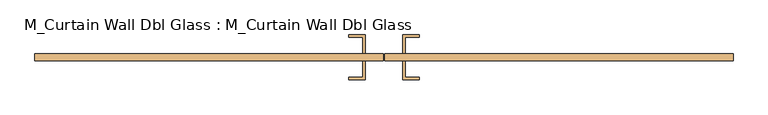
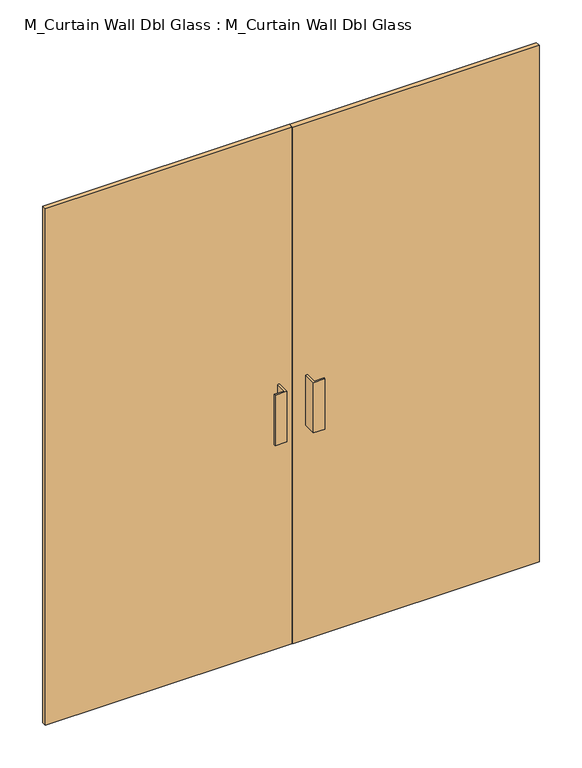
"""IFC4 building model written with IfcOpenShell, lengths in millimetres: door geometry, M_Curtain Wall Dbl Glass : M_Curtain Wall Dbl Glass."""

import ifcopenshell
import ifcopenshell.guid

model = None  # the IFC model being written
_history = None  # IfcOwnerHistory: only IFC2X3 demands one
_inside = {}  # id of a spatial element -> (the spatial element, [elements in it])
_under = {}  # id of a project, library or spatial element -> (it, [spatial elements below it])
_declared = {}  # id of a project -> (the project, [libraries it declares])
_typed = {}  # id of a type object -> (the type object, [elements of that type])
_made_of = {}  # id of a material, layer set ... -> (it, [elements and type objects made of it])


def new_model(schema):
    """Start an empty IFC model of exactly this schema.

    Asked for "IFC4X3", IfcOpenShell would pick the latest addendum, in which some entities
    have other attributes; the version numbers below select the first issue.
    IFC2X3 requires an IfcOwnerHistory on every rooted entity: one is made here for all.
    """
    global model, _history
    if schema == "IFC4X3":
        model = ifcopenshell.file(schema_version=(4, 3, 0, 0))
    else:
        model = ifcopenshell.file(schema=schema)
    _inside.clear()
    _under.clear()
    _declared.clear()
    _typed.clear()
    _made_of.clear()
    _history = None
    if model.schema == "IFC2X3":
        org = make("IfcOrganization", Name="unknown")
        user = make(
            "IfcPersonAndOrganization",
            ThePerson=make("IfcPerson", FamilyName="unknown"),
            TheOrganization=org,
        )
        app = make(
            "IfcApplication",
            ApplicationDeveloper=org,
            Version="unknown",
            ApplicationFullName="unknown",
            ApplicationIdentifier="unknown",
        )
        _history = make(
            "IfcOwnerHistory",
            OwningUser=user,
            OwningApplication=app,
            ChangeAction="ADDED",
            CreationDate=0,
        )
    return model


def make(cls, **values):
    """One entity of the class cls with the attributes given. An attribute that is None is left unset."""
    return model.create_entity(
        cls, **{name: value for name, value in values.items() if value is not None}
    )


def rooted(cls, **values):
    """An entity with a GlobalId (a new one), such as an element, a storey or a relation."""
    return make(cls, GlobalId=ifcopenshell.guid.new(), OwnerHistory=_history, **values)


def si_unit(unit_type, name, prefix=None):
    """IfcSIUnit, for example si_unit("LENGTHUNIT", "METRE", prefix="MILLI")."""
    return make("IfcSIUnit", UnitType=unit_type, Prefix=prefix, Name=name)


def assignment(units):
    """IfcUnitAssignment: the units of a project."""
    return None if units is None else make("IfcUnitAssignment", Units=units)


def point(xyz):
    """IfcCartesianPoint."""
    return None if xyz is None else make("IfcCartesianPoint", Coordinates=xyz)


def direction(xyz):
    """IfcDirection."""
    return None if xyz is None else make("IfcDirection", DirectionRatios=xyz)


def frame(location, z_axis=None, x_axis=None):
    """IfcAxis2Placement3D, a coordinate frame: its origin and axes. An axis left out is left unset."""
    return make(
        "IfcAxis2Placement3D",
        Location=point(location),
        Axis=direction(z_axis),
        RefDirection=direction(x_axis),
    )


def origin():
    """The frame at (0, 0, 0) with its axes left unset."""
    return frame((0.0, 0.0, 0.0))


def origin_with_axes():
    """The frame at (0, 0, 0) with the z axis (0, 0, 1) and the x axis (1, 0, 0) written out."""
    return frame((0.0, 0.0, 0.0), z_axis=(0.0, 0.0, 1.0), x_axis=(1.0, 0.0, 0.0))


def place(relative_to, where):
    """IfcLocalPlacement: puts the frame where relative to a parent placement (None: the world)."""
    return make(
        "IfcLocalPlacement", PlacementRelTo=relative_to, RelativePlacement=where
    )


def context(
    kind, dimensions, precision=None, world=None, true_north=None, identifier=None
):
    """IfcGeometricRepresentationContext, for example the 3D "Model" context."""
    return make(
        "IfcGeometricRepresentationContext",
        ContextIdentifier=identifier,
        ContextType=kind,
        CoordinateSpaceDimension=dimensions,
        Precision=precision,
        WorldCoordinateSystem=world,
        TrueNorth=true_north,
    )


def project(units=None, contexts=None):
    """IfcProject with its units and contexts."""
    return rooted(
        "IfcProject",
        Name="project",
        RepresentationContexts=contexts,
        UnitsInContext=assignment(units),
    )


def spatial(cls, under=None, at=None, **own):
    """A site, building, storey or space (cls), placed at a placement, below another one or the project."""
    s = rooted(cls, ObjectPlacement=at, **own)
    if under is not None:
        _under.setdefault(under.id(), (under, []))[1].append(s)
    return s


def polyline(points):
    """IfcPolyline through the points."""
    return make("IfcPolyline", Points=[point(p) for p in points])


def outline(outer, holes=None, kind="AREA"):
    """IfcArbitraryClosedProfileDef: a profile drawn as a closed curve; with holes, ...WithVoids."""
    if holes is None:
        return make("IfcArbitraryClosedProfileDef", ProfileType=kind, OuterCurve=outer)
    return make(
        "IfcArbitraryProfileDefWithVoids",
        ProfileType=kind,
        OuterCurve=outer,
        InnerCurves=holes,
    )


def extrude(swept, where, along, depth):
    """IfcExtrudedAreaSolid: the profile swept, set in the frame where, extruded along a direction by depth."""
    return make(
        "IfcExtrudedAreaSolid",
        SweptArea=swept,
        Position=where,
        ExtrudedDirection=direction(along),
        Depth=depth,
    )


def shape(context_of_items, identifier, shape_type, items):
    """IfcShapeRepresentation: the items that make up one representation, for example the "Body"."""
    return make(
        "IfcShapeRepresentation",
        ContextOfItems=context_of_items,
        RepresentationIdentifier=identifier,
        RepresentationType=shape_type,
        Items=items,
    )


def source(mapping_origin, context_of_items, identifier, shape_type, items):
    """IfcRepresentationMap: a shape defined once, which mapped items show again and again."""
    return make(
        "IfcRepresentationMap",
        MappingOrigin=mapping_origin,
        MappedRepresentation=shape(context_of_items, identifier, shape_type, items),
    )


def transform(
    local_origin,
    x_axis=None,
    y_axis=None,
    z_axis=None,
    scale=None,
    scale2=None,
    scale3=None,
    uniform=True,
):
    """IfcCartesianTransformationOperator3D, or its non-uniform kind. x_axis, y_axis, z_axis: its Axis1, 2, 3."""
    if uniform:
        return make(
            "IfcCartesianTransformationOperator3D",
            Axis1=direction(x_axis),
            Axis2=direction(y_axis),
            LocalOrigin=point(local_origin),
            Scale=scale,
            Axis3=direction(z_axis),
        )
    return make(
        "IfcCartesianTransformationOperator3DnonUniform",
        Axis1=direction(x_axis),
        Axis2=direction(y_axis),
        LocalOrigin=point(local_origin),
        Scale=scale,
        Axis3=direction(z_axis),
        Scale2=scale2,
        Scale3=scale3,
    )


def mapped(mapping_source, mapping_target):
    """IfcMappedItem: shows the shape of a source again, moved by a transform."""
    return make(
        "IfcMappedItem", MappingSource=mapping_source, MappingTarget=mapping_target
    )


def made_of(thing, what):
    """Note that an element or type object is made of a material, layer set ...; save() writes the relation."""
    if what is not None:
        _made_of.setdefault(what.id(), (what, []))[1].append(thing)
    return thing


def element(
    cls,
    number,
    at=None,
    inside=None,
    cuts=None,
    type_object=None,
    material=None,
    context=None,
    identifier="Body",
    shape_type=None,
    held_by="IfcProductDefinitionShape",
    body=None,
    shapes=None,
    **own,
):
    """One element of the class cls, such as IfcWall. Its Tag is "e" and its number.

    at: its placement. inside: the storey or other place that contains it. cuts: it is an
    opening in that element (IfcRelVoidsElement). A single representation is given by context,
    identifier, shape_type and body (its items); several are given by shapes. held_by: the class
    of the entity that holds the representations. save() writes the other relations.
    """
    e = rooted(cls, Tag="e%d" % number, ObjectPlacement=at, **own)
    if body is not None:
        shapes = [shape(context, identifier, shape_type, body)]
    if shapes is not None:
        e.Representation = make(held_by, Representations=shapes)
    if inside is not None:
        _inside.setdefault(inside.id(), (inside, []))[1].append(e)
    if cuts is not None:
        rooted(
            "IfcRelVoidsElement", RelatingBuildingElement=cuts, RelatedOpeningElement=e
        )
    if type_object is not None:
        _typed.setdefault(type_object.id(), (type_object, []))[1].append(e)
    return made_of(e, material)


def aggregate(whole, parts):
    """IfcRelAggregates: a whole, such as a stair, and the parts it consists of."""
    return rooted("IfcRelAggregates", RelatingObject=whole, RelatedObjects=parts)


def save(model, path):
    """Write the relations noted so far, then the file.

    IfcRelAggregates (storeys below a building ...), IfcRelContainedInSpatialStructure (elements
    in a storey), IfcRelDefinesByType, IfcRelAssociatesMaterial and IfcRelDeclares: one each for
    every whole, place, type object, material and project.
    """
    for whole, parts in _under.values():
        aggregate(whole, parts)
    for where, things in _inside.values():
        rooted(
            "IfcRelContainedInSpatialStructure",
            RelatedElements=things,
            RelatingStructure=where,
        )
    for kind, things in _typed.values():
        rooted("IfcRelDefinesByType", RelatedObjects=things, RelatingType=kind)
    for what, things in _made_of.values():
        rooted("IfcRelAssociatesMaterial", RelatedObjects=things, RelatingMaterial=what)
    for by, libraries in _declared.values():
        rooted("IfcRelDeclares", RelatingContext=by, RelatedDefinitions=libraries)
    model.write(path)


def m_curtain_wall_dbl_glass_m_curtain_wall_dbl_glass_0875745b(model_context):
    return source(origin(), model_context, "Body", "SweptSolid", [
        extrude(outline(polyline([(-1.5875, 30.95), (-942.5, 30.95), (-942.5, 50.0), (-1.5875, 50.0), (-1.5875, 30.95)])), origin_with_axes(), (0.0, 0.0, 1.0), 2085.0),
        extrude(outline(polyline([(942.5, 30.95), (1.5875, 30.95), (1.5875, 50.0), (942.5, 50.0), (942.5, 30.95)])), origin_with_axes(), (0.0, 0.0, 1.0), 2085.0),
        extrude(outline(polyline([(-50.8, 100.8), (-50.8, 50.0), (-57.15, 50.0), (-57.15, 94.45), (-95.25, 94.45), (-95.25, 100.8), (-50.8, 100.8)])), frame((0.0, 0.0, 863.6), z_axis=(0.0, 0.0, 1.0), x_axis=(1.0, 0.0, 0.0)), (0.0, 0.0, 1.0), 203.2),
        extrude(outline(polyline([(50.8, 100.8), (95.25, 100.8), (95.25, 94.45), (57.15, 94.45), (57.15, 50.0), (50.8, 50.0), (50.8, 100.8)])), frame((0.0, 0.0, 863.6), z_axis=(0.0, 0.0, 1.0), x_axis=(1.0, 0.0, 0.0)), (0.0, 0.0, 1.0), 203.2),
        extrude(outline(polyline([(-50.8, -19.85), (-95.25, -19.85), (-95.25, -13.5), (-57.15, -13.5), (-57.15, 30.95), (-50.8, 30.95), (-50.8, -19.85)])), frame((0.0, 0.0, 863.6), z_axis=(0.0, 0.0, 1.0), x_axis=(1.0, 0.0, 0.0)), (0.0, 0.0, 1.0), 203.2),
        extrude(outline(polyline([(50.8, -19.85), (50.8, 30.95), (57.15, 30.95), (57.15, -13.5), (95.25, -13.5), (95.25, -19.85), (50.8, -19.85)])), frame((0.0, 0.0, 863.6), z_axis=(0.0, 0.0, 1.0), x_axis=(1.0, 0.0, 0.0)), (0.0, 0.0, 1.0), 203.2),
    ])


if __name__ == "__main__":
    model = new_model("IFC4")
    model_context = context("Model", 3, world=origin())
    ifc_project = project(units=[si_unit("LENGTHUNIT", "METRE", prefix="MILLI")], contexts=[model_context])
    site = spatial("IfcSite", under=ifc_project)
    building = spatial("IfcBuilding", under=site)
    placement = place(None, origin())
    m_curtain_wall_dbl_glass_m_curtain_wall_dbl_glass_shape = m_curtain_wall_dbl_glass_m_curtain_wall_dbl_glass_0875745b(model_context)
    element("IfcDoor", 1, ObjectType="M_Curtain Wall Dbl Glass : M_Curtain Wall Dbl Glass", at=placement, inside=building, context=model_context, shape_type="MappedRepresentation", body=[
        mapped(m_curtain_wall_dbl_glass_m_curtain_wall_dbl_glass_shape, transform((0.0, 0.0, 0.0), x_axis=(1.0, 0.0, 0.0), y_axis=(0.0, 1.0, 0.0), z_axis=(0.0, 0.0, 1.0))),
    ])
    save(model, "model.ifc")

# Revit data of these elements
# Project information
#   Organization Name = "Eagle North America"
#   Organization Description = "Maximo demo data"
#   Building Name = "Executive Briefing Centerr"
#   Author = "design@eagle.com"
#   COBie.CreatedBy = "design@eagle.com"
#   COBie.CreatedOn = "2016-09-13T05:47:35"
#   COBie.Facility.Name = "Executive Briefing Centerr"
#   COBie.Facility.Category = "Eagle North America"
#   COBie.Facility.ProjectName = "Executive Briefing Centerr"
#   COBie.Facility.SiteName = "Valley Forge"
#   COBie.Facility.LinearUnits = "Millimeters"
#   COBie.Facility.AreaUnits = "Square Meters"
#   COBie.Facility.VolumeUnits = "Cubic Meters"
#   COBie.Facility.CurrencyUnit = "Dollar"
#   COBie.Facility.AreaMeasurement = "Revit Default Area Calculation Method"
#   COBie.Facility.Description = "Executive Briefing Centerr"
#   COBie.Facility.ProjectDescription = "Briefing Center build out in Lease space"
#   COBie.Facility.SiteDescription = "King of Prussia business center"
#   COBie.Facility.Phase = "Existing"
#   Project Issue Date = "2016-08-24"
#   Project Status = "Opertional"
#   Client Name = "Eagle North America"
#   Project Address = "1001 East Swedesford Road King of Prussia, PA 19406 USA"
#   Project Name = "Executive Briefing Centerr"
#   Project Number = "VF-21-15"
# Type "M_Curtain Wall Dbl Glass : M_Curtain Wall Dbl Glass"
#   Model = "12345678"
#   Manufacturer = "Dublin Doors"
#   Description = "Double Glass Door"
#   Type Mark = "41"
#   COBie.Type.CreatedBy = "design@eagle.com"
#   COBie.Type.CreatedOn = "2016-09-13T05:47:35"
#   COBie.Type.Name = "Doors_M_Curtain Wall Dbl Glass_M_Curtain Wall Dbl Glass"
#   COBie.Type.Category = "23-30 10 00 : Doors"
#   COBie.Type.Description = "Double Glass Door"
#   COBie.Type.Manufacturer = "Dublin Doors"
#   COBie.Type.ModelNumber = "12345678"
#   Construction Type Id = "GSP4R"
#   Analytic Construction = "1/8 in Pilkington single glazing"
#   COBie.Type.ReplacementCost = 0
#   Visual Light Transmittance = 0.9
#   Solar Heat Gain Coefficient = 0.78
#   Offset = 50 mm
#   Heat Transfer Coefficient (U) = 3.6886 W/(m²·K)
#   COBie.Type = yes
#   Function = 1
#   Glazing Material = Glass
# Element 1 (IfcDoor, "M_Curtain Wall Dbl Glass : M_Curtain Wall Dbl Glass")
#   Materials on its faces: "Aluminum", "Glass"
# Materials
#   "Glass": class "Glass", colour RGB 0 128 192, transparency 0.75, Description = "Soda Lime Glass", Cost = 0
#   "Aluminum": class "Metal", colour RGB 247 247 247, transparency 0, Description = "Aluminum 6061", Cost = 0
